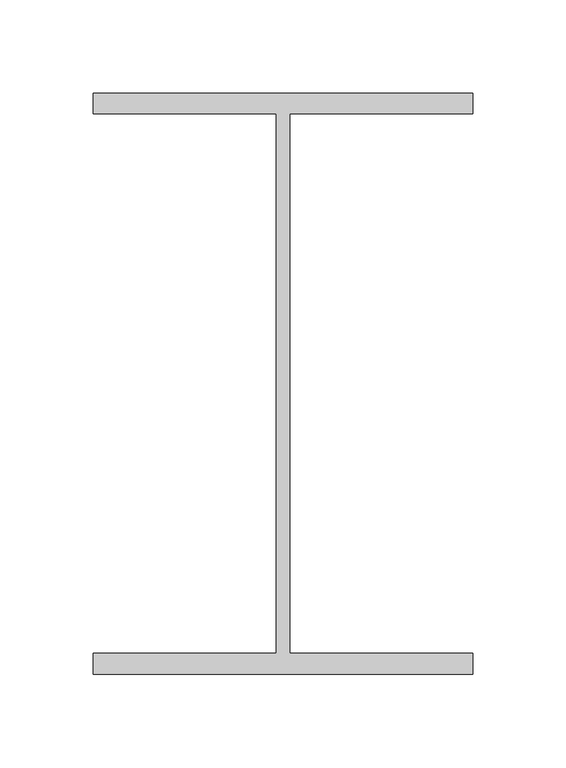
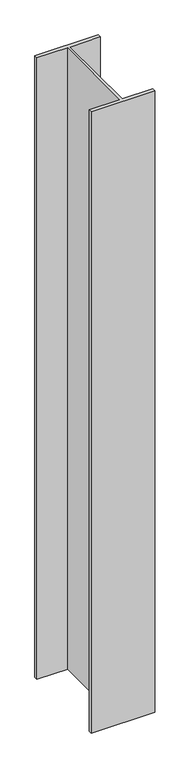
"""IFC4 building model written with IfcOpenShell, lengths in millimetres: proxy geometry, Generic Models 2:Generic Models 2:310765:Generic Models 2:310765 : Generic Models 2:Generic Models 2:310765:202 : Generic Models 2:Generic Models 2:310765:Generic Models 2:310765 : Generic Models 2:Generic Models 2:310765:300385."""

from ifc_helpers import new_model, si_unit, frame, origin, place, context, project, spatial, polyline, outline, extrude, source, transform, mapped, element, save


def generic_models_2755017a(model_context):
    return source(origin(), model_context, "Body", "SweptSolid", [
        extrude(outline(polyline([(579104.5117239, -567621.4913841), (579104.5117239, -567632.5046653), (579006.5828177, -567632.5046653), (579006.5828177, -567921.6281028), (579104.5117239, -567921.6281028), (579104.5117239, -567932.6413841), (578901.2863239, -567932.6413841), (578901.2863239, -567921.6281028), (578999.2406302, -567921.6281028), (578999.2406302, -567632.5046653), (578901.3117239, -567632.5046653), (578901.3117239, -567621.4913841), (579104.5117239, -567621.4913841)])), frame((0.0, 0.0, 4033.8810286), z_axis=(0.0, 0.0, 1.0), x_axis=(1.0, 0.0, 0.0)), (0.0, 0.0, 1.0), 2100.2189714),
    ])


if __name__ == "__main__":
    model = new_model("IFC4")
    model_context = context("Model", 3, world=origin())
    ifc_project = project(units=[si_unit("LENGTHUNIT", "METRE", prefix="MILLI")], contexts=[model_context])
    site = spatial("IfcSite", under=ifc_project)
    building = spatial("IfcBuilding", under=site)
    placement = place(None, origin())
    generic_models_shape = generic_models_2755017a(model_context)
    element("IfcBuildingElementProxy", 1, Name="Generic Models 2:Generic Models 2:310765:Generic Models 2:310765 : Generic Models 2:Generic Models 2:310765:202 : Generic Models 2:Generic Models 2:310765:Generic Models 2:310765 : Generic Models 2:Generic Models 2:310765:300385", ObjectType="Generic Models 2:Generic Models 2:310765:Generic Models 2:310765 : Generic Models 2:Generic Models 2:310765:202 : Generic Models 2:Generic Models 2:310765:Generic Models 2:310765 : Generic Models 2:Generic Models 2:310765:300385", at=placement, inside=building, context=model_context, shape_type="MappedRepresentation", body=[
        mapped(generic_models_shape, transform((0.0, 0.0, 0.0), x_axis=(1.0, 0.0, 0.0), y_axis=(0.0, 1.0, 0.0), z_axis=(0.0, 0.0, 1.0))),
    ])
    save(model, "model.ifc")

# Revit data of these elements
# Type "Generic Models 2:Generic Models 2:310765:Generic Models 2:310765 : Generic Models 2:Generic Models 2:310765:202 : Generic Models 2:Generic Models 2:310765:Generic Models 2:310765 : Generic Models 2:Generic Models 2:310765:300385"
#   NameOverride = "Generic Models 2:Generic Models 2:310765:Generic Models 2:310765 : Generic Models 2:Generic Models 2:310765:300385"
#   ObjectTypeOverride = "Generic Models 2:310765 : Generic Models 2:Generic Models 2:310765"
#   Reference = "Generic Models 2"
#   Tag = "300385"
# Element 1 (IfcBuildingElementProxy, "Generic Models 2:Generic Models 2:310765:Generic Models 2:310765 : Generic Models 2:Generic Models 2:310765:202 : Generic Models 2:Generic Models 2:310765:Generic Models 2:310765 : Generic Models 2:Generic Models 2:310765:300385")
#   Materials on its faces: "STRUCTURAL STEEL - SEE STRUCT. DWGS"
# Materials
#   "STRUCTURAL STEEL - SEE STRUCT. DWGS": class "Metal", colour RGB 189 187 185, transparency 0, Description = "Structural steel 50ksi", Cost = 0
